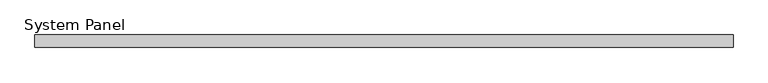
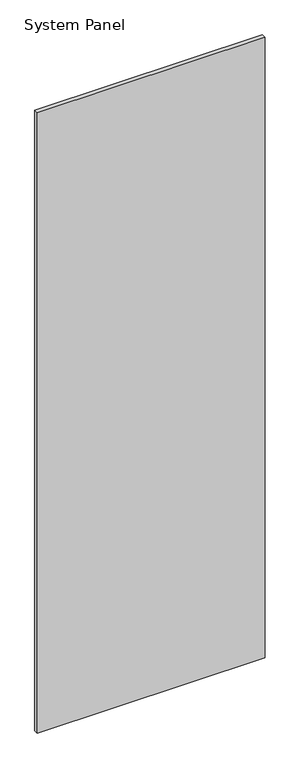
"""IFC4 building model written with IfcOpenShell, lengths in millimetres: plate geometry, System Panel : WWm-Glass-20mm-10mmOffset."""

from ifc_helpers import new_model, si_unit, origin, origin_with_axes, place, context, project, spatial, polyline, outline, extrude, source, transform, mapped, element, save


def system_panel_7f9515ec(model_context):
    return source(origin(), model_context, "Body", "SweptSolid", [
        extrude(outline(polyline([(565.0, 0.0), (-565.0, 0.0), (-565.0, 20.0), (565.0, 20.0), (565.0, 0.0)])), origin_with_axes(), (0.0, 0.0, 1.0), 3250.0),
    ])


if __name__ == "__main__":
    model = new_model("IFC4")
    model_context = context("Model", 3, world=origin())
    ifc_project = project(units=[si_unit("LENGTHUNIT", "METRE", prefix="MILLI")], contexts=[model_context])
    site = spatial("IfcSite", under=ifc_project)
    building = spatial("IfcBuilding", under=site)
    placement = place(None, origin())
    system_panel_shape = system_panel_7f9515ec(model_context)
    element("IfcPlate", 1, ObjectType="System Panel : WWm-Glass-20mm-10mmOffset", at=placement, inside=building, context=model_context, shape_type="MappedRepresentation", body=[
        mapped(system_panel_shape, transform((0.0, 0.0, 0.0), x_axis=(1.0, 0.0, 0.0), y_axis=(0.0, 1.0, 0.0), z_axis=(0.0, 0.0, 1.0))),
    ])
    save(model, "model.ifc")

# Revit data of these elements
# Type "System Panel : WWm-Glass-20mm-10mmOffset"
#   Finish = ""
# Element 1 (IfcPlate, "System Panel : WWm-Glass-20mm-10mmOffset")
#   Materials on its faces: "WW-EC-GL-Storefront"
# Materials
#   "WW-EC-GL-Storefront": class "Glass", colour RGB 236 240 239, transparency 0.85, Description = "Storefront Glass", Cost = 0
